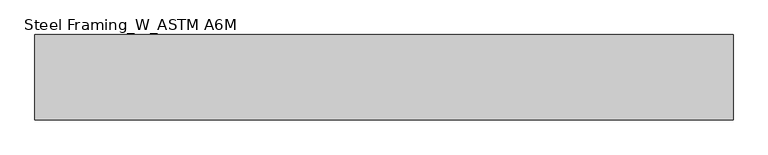
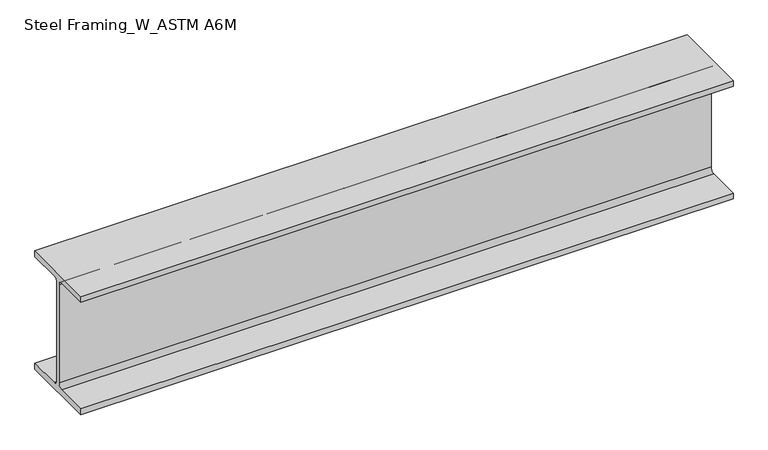
"""IFC4 building model written with IfcOpenShell, lengths in millimetres: beam geometry, Steel Framing_W_ASTM A6M : H_SB_AR_S02_W200x31.3_B6."""

from ifc_helpers import new_model, si_unit, point, frame, frame_2d, origin, place, context, project, spatial, polyline, circle_curve, trimmed, segment, composite_curve, outline, extrude, source, transform, mapped, element, save


def steel_framing_w_astm_a6m_519ed75d(model_context):
    return source(origin(), model_context, "Body", "SweptSolid", [
        extrude(outline(composite_curve([segment(polyline([(67.0, -94.8), (67.0, -105.0), (-67.0, -105.0), (-67.0, -94.8), (-10.775, -94.8)]), True, "CONTINUOUS"), segment(trimmed(circle_curve(frame_2d((-10.775, -87.2)), 7.6), [point((-10.775, -94.8))], [point((-3.175, -87.2))], True, "CARTESIAN"), True, "CONTINUOUS"), segment(polyline([(-3.175, -87.2), (-3.175, 87.2)]), True, "CONTINUOUS"), segment(trimmed(circle_curve(frame_2d((-10.775, 87.2)), 7.6), [point((-3.175, 87.2))], [point((-10.775, 94.8))], True, "CARTESIAN"), True, "CONTINUOUS"), segment(polyline([(-10.775, 94.8), (-67.0, 94.8), (-67.0, 105.0), (67.0, 105.0), (67.0, 94.8), (10.775, 94.8)]), True, "CONTINUOUS"), segment(trimmed(circle_curve(frame_2d((10.775, 87.2)), 7.6), [point((10.775, 94.8))], [point((3.175, 87.2))], True, "CARTESIAN"), True, "CONTINUOUS"), segment(polyline([(3.175, 87.2), (3.175, -87.2)]), True, "CONTINUOUS"), segment(trimmed(circle_curve(frame_2d((10.775, -87.2)), 7.6), [point((3.175, -87.2))], [point((10.775, -94.8))], True, "CARTESIAN"), True, "CONTINUOUS"), segment(polyline([(10.775, -94.8), (67.0, -94.8)]), True, "CONTINUOUS")], self_intersect=False)), frame((-585.3, 0.0, 0.0), z_axis=(1.0, 0.0, 0.0), x_axis=(0.0, 1.0, 0.0)), (0.0, 0.0, 1.0), 1096.6),
    ])


if __name__ == "__main__":
    model = new_model("IFC4")
    model_context = context("Model", 3, world=origin())
    ifc_project = project(units=[si_unit("LENGTHUNIT", "METRE", prefix="MILLI")], contexts=[model_context])
    site = spatial("IfcSite", under=ifc_project)
    building = spatial("IfcBuilding", under=site)
    placement = place(None, origin())
    steel_framing_w_astm_a6m_shape = steel_framing_w_astm_a6m_519ed75d(model_context)
    element("IfcBeam", 1, ObjectType="Steel Framing_W_ASTM A6M : H_SB_AR_S02_W200x31.3_B6", at=placement, inside=building, context=model_context, shape_type="MappedRepresentation", body=[
        mapped(steel_framing_w_astm_a6m_shape, transform((0.0, 0.0, 0.0), x_axis=(1.0, 0.0, 0.0), y_axis=(0.0, 1.0, 0.0), z_axis=(0.0, 0.0, 1.0))),
    ])
    save(model, "model.ifc")

# Revit data of these elements
# Type "Steel Framing_W_ASTM A6M : H_SB_AR_S02_W200x31.3_B6"
#   Type Mark = "B6"
#   Section Name Key = "W8x21"
#   Width = 13.4 cm
#   Web Thickness = 0.635 cm
#   Web Fillet = 0.76 cm
#   Warping Constant = 40800.0 cm⁶
#   Torsional Moment of Inertia = 11.70 cm⁴
#   Section Area = 39.7 cm²
#   Plastic Modulus weak axis = 93.2 cm³
#   Plastic Modulus strong axis = 334.0 cm³
#   Perimeter = 0.93 m²/m
#   Nominal Weight = 31.30 kgf/m
#   Moment of Inertia weak axis = 407.00 cm⁴
#   Moment of Inertia strong axis = 3130.00 cm⁴
#   Height = 21.0 cm
#   Flange Thickness = 1.02 cm
#   Elastic Modulus weak axis = 60.8 cm³
#   Elastic Modulus strong axis = 298.0 cm³
#   Centroid Vertical = 10.5 cm
#   Centroid Horizontal = 6.7 cm
#   Length [instance default] = 1500 mm
#   Structural Material [instance default] = Steel, 45-345
#   Bolt Spacing = 0
#   Assembly Code = ""
# Element 1 (IfcBeam, "Steel Framing_W_ASTM A6M : H_SB_AR_S02_W200x31.3_B6")
#   Materials on its faces: "Steel, 45-345"
# Materials
#   "Steel, 45-345": class "Metal", colour RGB 189 187 185, transparency 0, Description = "Steel 345 MPa", Cost = 0
